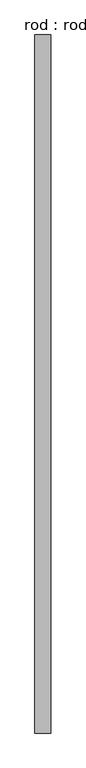
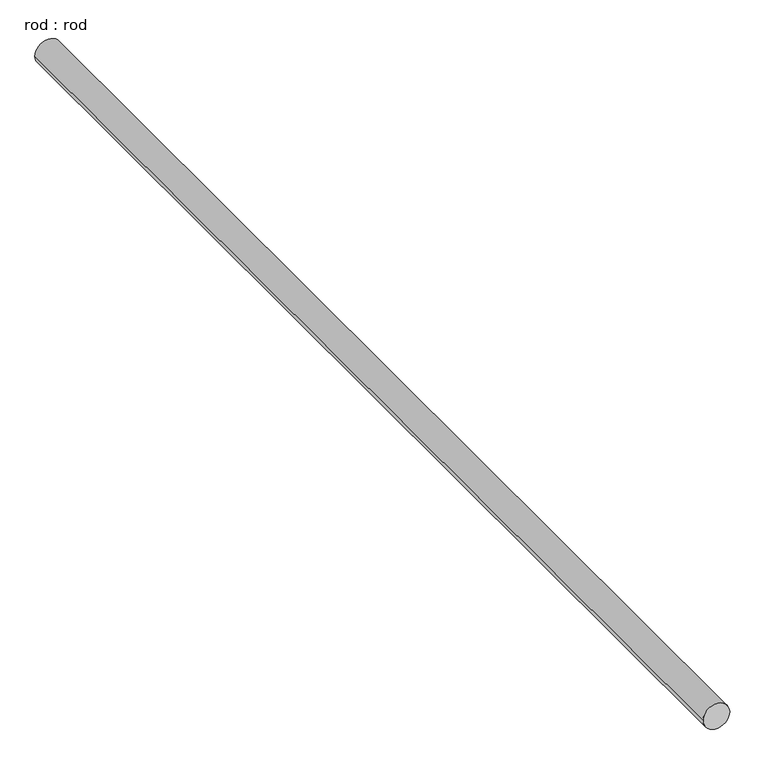
"""IFC4 building model written with IfcOpenShell, lengths in millimetres: proxy geometry, rod : rod."""

import ifcopenshell
import ifcopenshell.guid

model = None  # the IFC model being written
_history = None  # IfcOwnerHistory: only IFC2X3 demands one
_inside = {}  # id of a spatial element -> (the spatial element, [elements in it])
_under = {}  # id of a project, library or spatial element -> (it, [spatial elements below it])
_declared = {}  # id of a project -> (the project, [libraries it declares])
_typed = {}  # id of a type object -> (the type object, [elements of that type])
_made_of = {}  # id of a material, layer set ... -> (it, [elements and type objects made of it])


def new_model(schema):
    """Start an empty IFC model of exactly this schema.

    Asked for "IFC4X3", IfcOpenShell would pick the latest addendum, in which some entities
    have other attributes; the version numbers below select the first issue.
    IFC2X3 requires an IfcOwnerHistory on every rooted entity: one is made here for all.
    """
    global model, _history
    if schema == "IFC4X3":
        model = ifcopenshell.file(schema_version=(4, 3, 0, 0))
    else:
        model = ifcopenshell.file(schema=schema)
    _inside.clear()
    _under.clear()
    _declared.clear()
    _typed.clear()
    _made_of.clear()
    _history = None
    if model.schema == "IFC2X3":
        org = make("IfcOrganization", Name="unknown")
        user = make(
            "IfcPersonAndOrganization",
            ThePerson=make("IfcPerson", FamilyName="unknown"),
            TheOrganization=org,
        )
        app = make(
            "IfcApplication",
            ApplicationDeveloper=org,
            Version="unknown",
            ApplicationFullName="unknown",
            ApplicationIdentifier="unknown",
        )
        _history = make(
            "IfcOwnerHistory",
            OwningUser=user,
            OwningApplication=app,
            ChangeAction="ADDED",
            CreationDate=0,
        )
    return model


def make(cls, **values):
    """One entity of the class cls with the attributes given. An attribute that is None is left unset."""
    return model.create_entity(
        cls, **{name: value for name, value in values.items() if value is not None}
    )


def rooted(cls, **values):
    """An entity with a GlobalId (a new one), such as an element, a storey or a relation."""
    return make(cls, GlobalId=ifcopenshell.guid.new(), OwnerHistory=_history, **values)


def si_unit(unit_type, name, prefix=None):
    """IfcSIUnit, for example si_unit("LENGTHUNIT", "METRE", prefix="MILLI")."""
    return make("IfcSIUnit", UnitType=unit_type, Prefix=prefix, Name=name)


def assignment(units):
    """IfcUnitAssignment: the units of a project."""
    return None if units is None else make("IfcUnitAssignment", Units=units)


def point(xyz):
    """IfcCartesianPoint."""
    return None if xyz is None else make("IfcCartesianPoint", Coordinates=xyz)


def direction(xyz):
    """IfcDirection."""
    return None if xyz is None else make("IfcDirection", DirectionRatios=xyz)


def frame(location, z_axis=None, x_axis=None):
    """IfcAxis2Placement3D, a coordinate frame: its origin and axes. An axis left out is left unset."""
    return make(
        "IfcAxis2Placement3D",
        Location=point(location),
        Axis=direction(z_axis),
        RefDirection=direction(x_axis),
    )


def frame_2d(location, x_axis=None):
    """IfcAxis2Placement2D, a coordinate frame in the plane: its origin and x axis."""
    return make(
        "IfcAxis2Placement2D", Location=point(location), RefDirection=direction(x_axis)
    )


def origin():
    """The frame at (0, 0, 0) with its axes left unset."""
    return frame((0.0, 0.0, 0.0))


def place(relative_to, where):
    """IfcLocalPlacement: puts the frame where relative to a parent placement (None: the world)."""
    return make(
        "IfcLocalPlacement", PlacementRelTo=relative_to, RelativePlacement=where
    )


def context(
    kind, dimensions, precision=None, world=None, true_north=None, identifier=None
):
    """IfcGeometricRepresentationContext, for example the 3D "Model" context."""
    return make(
        "IfcGeometricRepresentationContext",
        ContextIdentifier=identifier,
        ContextType=kind,
        CoordinateSpaceDimension=dimensions,
        Precision=precision,
        WorldCoordinateSystem=world,
        TrueNorth=true_north,
    )


def project(units=None, contexts=None):
    """IfcProject with its units and contexts."""
    return rooted(
        "IfcProject",
        Name="project",
        RepresentationContexts=contexts,
        UnitsInContext=assignment(units),
    )


def spatial(cls, under=None, at=None, **own):
    """A site, building, storey or space (cls), placed at a placement, below another one or the project."""
    s = rooted(cls, ObjectPlacement=at, **own)
    if under is not None:
        _under.setdefault(under.id(), (under, []))[1].append(s)
    return s


def circle_curve(where, radius):
    """IfcCircle in the frame where."""
    return make("IfcCircle", Position=where, Radius=radius)


def trimmed(basis, trim1, trim2, sense, master):
    """IfcTrimmedCurve: the piece of a basis curve between two trims."""
    return make(
        "IfcTrimmedCurve",
        BasisCurve=basis,
        Trim1=trim1,
        Trim2=trim2,
        SenseAgreement=sense,
        MasterRepresentation=master,
    )


def segment(curve, same_sense, transition):
    """IfcCompositeCurveSegment."""
    return make(
        "IfcCompositeCurveSegment",
        Transition=transition,
        SameSense=same_sense,
        ParentCurve=curve,
    )


def composite_curve(segments, self_intersect=None):
    """IfcCompositeCurve: segments joined end to end."""
    return make("IfcCompositeCurve", Segments=segments, SelfIntersect=self_intersect)


def outline(outer, holes=None, kind="AREA"):
    """IfcArbitraryClosedProfileDef: a profile drawn as a closed curve; with holes, ...WithVoids."""
    if holes is None:
        return make("IfcArbitraryClosedProfileDef", ProfileType=kind, OuterCurve=outer)
    return make(
        "IfcArbitraryProfileDefWithVoids",
        ProfileType=kind,
        OuterCurve=outer,
        InnerCurves=holes,
    )


def extrude(swept, where, along, depth):
    """IfcExtrudedAreaSolid: the profile swept, set in the frame where, extruded along a direction by depth."""
    return make(
        "IfcExtrudedAreaSolid",
        SweptArea=swept,
        Position=where,
        ExtrudedDirection=direction(along),
        Depth=depth,
    )


def shape(context_of_items, identifier, shape_type, items):
    """IfcShapeRepresentation: the items that make up one representation, for example the "Body"."""
    return make(
        "IfcShapeRepresentation",
        ContextOfItems=context_of_items,
        RepresentationIdentifier=identifier,
        RepresentationType=shape_type,
        Items=items,
    )


def source(mapping_origin, context_of_items, identifier, shape_type, items):
    """IfcRepresentationMap: a shape defined once, which mapped items show again and again."""
    return make(
        "IfcRepresentationMap",
        MappingOrigin=mapping_origin,
        MappedRepresentation=shape(context_of_items, identifier, shape_type, items),
    )


def transform(
    local_origin,
    x_axis=None,
    y_axis=None,
    z_axis=None,
    scale=None,
    scale2=None,
    scale3=None,
    uniform=True,
):
    """IfcCartesianTransformationOperator3D, or its non-uniform kind. x_axis, y_axis, z_axis: its Axis1, 2, 3."""
    if uniform:
        return make(
            "IfcCartesianTransformationOperator3D",
            Axis1=direction(x_axis),
            Axis2=direction(y_axis),
            LocalOrigin=point(local_origin),
            Scale=scale,
            Axis3=direction(z_axis),
        )
    return make(
        "IfcCartesianTransformationOperator3DnonUniform",
        Axis1=direction(x_axis),
        Axis2=direction(y_axis),
        LocalOrigin=point(local_origin),
        Scale=scale,
        Axis3=direction(z_axis),
        Scale2=scale2,
        Scale3=scale3,
    )


def mapped(mapping_source, mapping_target):
    """IfcMappedItem: shows the shape of a source again, moved by a transform."""
    return make(
        "IfcMappedItem", MappingSource=mapping_source, MappingTarget=mapping_target
    )


def made_of(thing, what):
    """Note that an element or type object is made of a material, layer set ...; save() writes the relation."""
    if what is not None:
        _made_of.setdefault(what.id(), (what, []))[1].append(thing)
    return thing


def element(
    cls,
    number,
    at=None,
    inside=None,
    cuts=None,
    type_object=None,
    material=None,
    context=None,
    identifier="Body",
    shape_type=None,
    held_by="IfcProductDefinitionShape",
    body=None,
    shapes=None,
    **own,
):
    """One element of the class cls, such as IfcWall. Its Tag is "e" and its number.

    at: its placement. inside: the storey or other place that contains it. cuts: it is an
    opening in that element (IfcRelVoidsElement). A single representation is given by context,
    identifier, shape_type and body (its items); several are given by shapes. held_by: the class
    of the entity that holds the representations. save() writes the other relations.
    """
    e = rooted(cls, Tag="e%d" % number, ObjectPlacement=at, **own)
    if body is not None:
        shapes = [shape(context, identifier, shape_type, body)]
    if shapes is not None:
        e.Representation = make(held_by, Representations=shapes)
    if inside is not None:
        _inside.setdefault(inside.id(), (inside, []))[1].append(e)
    if cuts is not None:
        rooted(
            "IfcRelVoidsElement", RelatingBuildingElement=cuts, RelatedOpeningElement=e
        )
    if type_object is not None:
        _typed.setdefault(type_object.id(), (type_object, []))[1].append(e)
    return made_of(e, material)


def aggregate(whole, parts):
    """IfcRelAggregates: a whole, such as a stair, and the parts it consists of."""
    return rooted("IfcRelAggregates", RelatingObject=whole, RelatedObjects=parts)


def save(model, path):
    """Write the relations noted so far, then the file.

    IfcRelAggregates (storeys below a building ...), IfcRelContainedInSpatialStructure (elements
    in a storey), IfcRelDefinesByType, IfcRelAssociatesMaterial and IfcRelDeclares: one each for
    every whole, place, type object, material and project.
    """
    for whole, parts in _under.values():
        aggregate(whole, parts)
    for where, things in _inside.values():
        rooted(
            "IfcRelContainedInSpatialStructure",
            RelatedElements=things,
            RelatingStructure=where,
        )
    for kind, things in _typed.values():
        rooted("IfcRelDefinesByType", RelatedObjects=things, RelatingType=kind)
    for what, things in _made_of.values():
        rooted("IfcRelAssociatesMaterial", RelatedObjects=things, RelatingMaterial=what)
    for by, libraries in _declared.values():
        rooted("IfcRelDeclares", RelatingContext=by, RelatedDefinitions=libraries)
    model.write(path)


def rod_rod_d9791cce(model_context):
    return source(origin(), model_context, "Body", "SweptSolid", [
        extrude(outline(composite_curve([segment(trimmed(circle_curve(frame_2d((0.0108462, 0.0)), 200.0), [point((0.0108462, 200.0))], [point((0.0108462, -200.0))], False, "CARTESIAN"), True, "CONTINUOUS"), segment(trimmed(circle_curve(frame_2d((0.0108462, 0.0)), 200.0), [point((0.0108462, -200.0))], [point((0.0108462, 200.0))], False, "CARTESIAN"), True, "CONTINUOUS")], self_intersect=False)), frame((0.0, -4636.2081137, 0.0), z_axis=(0.0, 1.0, 0.0), x_axis=(0.0, 0.0, 1.0)), (0.0, 0.0, 1.0), 17457.8734581),
    ])


if __name__ == "__main__":
    model = new_model("IFC4")
    model_context = context("Model", 3, world=origin())
    ifc_project = project(units=[si_unit("LENGTHUNIT", "METRE", prefix="MILLI")], contexts=[model_context])
    site = spatial("IfcSite", under=ifc_project)
    building = spatial("IfcBuilding", under=site)
    placement = place(None, origin())
    rod_rod_shape = rod_rod_d9791cce(model_context)
    element("IfcBuildingElementProxy", 1, Name="rod : rod", ObjectType="rod : rod", at=placement, inside=building, context=model_context, shape_type="MappedRepresentation", body=[
        mapped(rod_rod_shape, transform((0.0, 0.0, 0.0), x_axis=(1.0, 0.0, 0.0), y_axis=(0.0, 1.0, 0.0), z_axis=(0.0, 0.0, 1.0))),
    ])
    save(model, "model.ifc")

# Revit data of these elements
# Type "rod : rod"
#   Default Elevation = 0
